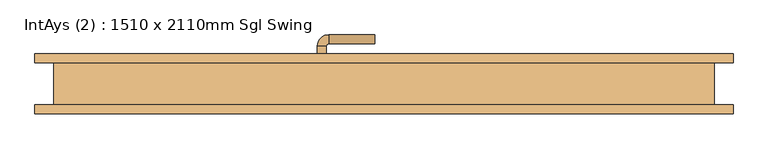
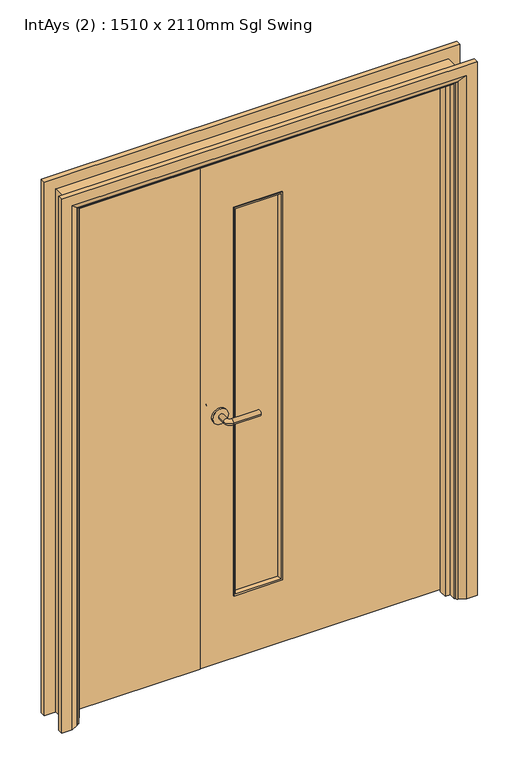
"""IFC4 building model written with IfcOpenShell, lengths in millimetres: door geometry, IntAys (2) : 1510 x 2110mm Sgl Swing."""

from ifc_helpers import new_model, si_unit, point, frame, frame_2d, origin, place, context, project, spatial, polyline, circle_curve, ellipse_curve, trimmed, segment, composite_curve, outline, extrude, faceted_brep, source, transform, mapped, element, save
from ifc_brep_helpers import plane_surface, cylinder_surface, revolved_surface, advanced_brep


def intays_2_1510_x_2110mm_sgl_swing_f165abe8(model_context):
    return source(origin(), model_context, "Body", "SolidModel", [
        advanced_brep(
        [(88.5, 7.5, 1000.0), (108.5, 7.5, 1000.0), (108.5, -22.5, 1000.0), (88.5, -22.5, 1000.0), (113.5, -27.5, 1000.0), (113.5, -47.5, 1000.0), (218.5, -47.5, 1000.0), (218.5, -27.5, 1000.0)],
        [
            (0, 1, circle_curve(frame((98.5, 7.5, 1000.0), z_axis=(0.0, 1.0, 0.0), x_axis=(1.0, 0.0, 0.0)), 10.0)),
            (1, 0, circle_curve(frame((98.5, 7.5, 1000.0), z_axis=(0.0, 1.0, 0.0), x_axis=(1.0, 0.0, 0.0)), 10.0)),
            (1, 2),
            (2, 3, circle_curve(frame((98.5, -22.5, 1000.0), z_axis=(0.0, 1.0, 0.0), x_axis=(1.0, 0.0, 0.0)), 10.0)),
            (3, 0),
            (3, 2, circle_curve(frame((98.5, -22.5, 1000.0), z_axis=(0.0, 1.0, 0.0), x_axis=(1.0, 0.0, 0.0)), 10.0)),
            (4, 5, circle_curve(frame((113.5, -37.5, 1000.0), z_axis=(-1.0, 0.0, 0.0), x_axis=(0.0, 1.0, 0.0)), 10.0)),
            (5, 3, circle_curve(frame((113.5, -22.5, 1000.0), z_axis=(0.0, 0.0, -1.0), x_axis=(-1.0, 0.0, 0.0)), 25.0)),
            (2, 4, circle_curve(frame((113.5, -22.5, 1000.0), z_axis=(0.0, 0.0, 1.0), x_axis=(-1.0, 0.0, 0.0)), 5.0)),
            (5, 4, circle_curve(frame((113.5, -37.5, 1000.0), z_axis=(-1.0, 0.0, 0.0), x_axis=(0.0, 1.0, 0.0)), 10.0)),
            (6, 7, circle_curve(frame((218.5, -37.5, 1000.0), z_axis=(1.0, 0.0, 0.0), x_axis=(0.0, 1.0, 0.0)), 10.0)),
            (7, 6, circle_curve(frame((218.5, -37.5, 1000.0), z_axis=(1.0, 0.0, 0.0), x_axis=(0.0, 1.0, 0.0)), 10.0)),
            (4, 7),
            (6, 5),
        ],
        [
            plane_surface(frame((98.5, 7.5, 1000.0), z_axis=(0.0, 1.0, 0.0), x_axis=(0.0, 0.0, 1.0))),
            cylinder_surface(frame((98.5, 7.5, 1000.0), z_axis=(0.0, 1.0, 0.0), x_axis=(1.0, 0.0, 0.0)), 10.0),
            revolved_surface(trimmed(ellipse_curve(frame((98.5, -22.5, 1000.0), z_axis=(0.0, -1.0, 0.0), x_axis=(1.0, 0.0, 0.0)), 10.0, 10.0), [point((88.5, -22.5, 1000.0))], [point((108.5, -22.5, 1000.0))], True, "CARTESIAN"), (113.5, -22.5, 1000.0), (0.0, 0.0, -1.0)),
            revolved_surface(trimmed(ellipse_curve(frame((98.5, -22.5, 1000.0), z_axis=(0.0, -1.0, 0.0), x_axis=(1.0, 0.0, 0.0)), 10.0, 10.0), [point((108.5, -22.5, 1000.0))], [point((88.5, -22.5, 1000.0))], True, "CARTESIAN"), (113.5, -22.5, 1000.0), (0.0, 0.0, -1.0)),
            plane_surface(frame((218.5, -37.5, 1000.0), z_axis=(1.0, 0.0, 0.0), x_axis=(0.0, 0.0, 1.0))),
            cylinder_surface(frame((113.5, -37.5, 1000.0), z_axis=(-1.0, 0.0, 0.0), x_axis=(0.0, 1.0, 0.0)), 10.0),
        ],
        [
            (0, [[1, 2]]),
            (1, [[3, 4, 5, -2]]),
            (1, [[-5, 6, -3, -1]]),
            (2, [[7, 8, -4, 9]]),
            (3, [[10, -9, -6, -8]]),
            (4, [[11, 12]]),
            (5, [[13, -11, 14, -7]]),
            (5, [[-14, -12, -13, -10]]),
        ],
    ),
        extrude(outline(composite_curve([segment(trimmed(circle_curve(frame_2d((1000.0, 96.0)), 30.0), [point((1000.0, 66.0))], [point((1000.0, 126.0))], False, "CARTESIAN"), True, "CONTINUOUS"), segment(trimmed(circle_curve(frame_2d((1000.0, 96.0)), 30.0), [point((1000.0, 126.0))], [point((1000.0, 66.0))], False, "CARTESIAN"), True, "CONTINUOUS")], self_intersect=False)), frame((0.0, 7.5, 0.0), z_axis=(0.0, 1.0, 0.0), x_axis=(0.0, 0.0, 1.0)), (0.0, 0.0, 1.0), 8.0),
        advanced_brep(
        [(88.5, 55.5, 1000.0), (108.5, 55.5, 1000.0), (88.5, 85.5, 1000.0), (108.5, 85.5, 1000.0), (113.5, 90.5, 1000.0), (113.5, 110.5, 1000.0), (218.5, 110.5, 1000.0), (218.5, 90.5, 1000.0)],
        [
            (0, 1, circle_curve(frame((98.5, 55.5, 1000.0), z_axis=(0.0, -1.0, 0.0), x_axis=(1.0, 0.0, 0.0)), 10.0)),
            (1, 0, circle_curve(frame((98.5, 55.5, 1000.0), z_axis=(0.0, -1.0, 0.0), x_axis=(1.0, 0.0, 0.0)), 10.0)),
            (0, 2),
            (2, 3, circle_curve(frame((98.5, 85.5, 1000.0), z_axis=(0.0, -1.0, 0.0), x_axis=(1.0, 0.0, 0.0)), 10.0)),
            (3, 1),
            (3, 2, circle_curve(frame((98.5, 85.5, 1000.0), z_axis=(0.0, -1.0, 0.0), x_axis=(1.0, 0.0, 0.0)), 10.0)),
            (4, 3, circle_curve(frame((113.5, 85.5, 1000.0), z_axis=(0.0, 0.0, 1.0), x_axis=(-1.0, 0.0, 0.0)), 5.0)),
            (2, 5, circle_curve(frame((113.5, 85.5, 1000.0), z_axis=(0.0, 0.0, -1.0), x_axis=(-1.0, 0.0, 0.0)), 25.0)),
            (5, 4, circle_curve(frame((113.5, 100.5, 1000.0), z_axis=(-1.0, 0.0, 0.0), x_axis=(0.0, -1.0, 0.0)), 10.0)),
            (4, 5, circle_curve(frame((113.5, 100.5, 1000.0), z_axis=(-1.0, 0.0, 0.0), x_axis=(0.0, -1.0, 0.0)), 10.0)),
            (6, 7, circle_curve(frame((218.5, 100.5, 1000.0), z_axis=(1.0, 0.0, 0.0), x_axis=(0.0, -1.0, 0.0)), 10.0)),
            (7, 6, circle_curve(frame((218.5, 100.5, 1000.0), z_axis=(1.0, 0.0, 0.0), x_axis=(0.0, -1.0, 0.0)), 10.0)),
            (5, 6),
            (7, 4),
        ],
        [
            plane_surface(frame((98.5, 55.5, 1000.0), z_axis=(0.0, -1.0, 0.0), x_axis=(0.0, 0.0, 1.0))),
            cylinder_surface(frame((98.5, 55.5, 1000.0), z_axis=(0.0, -1.0, 0.0), x_axis=(1.0, 0.0, 0.0)), 10.0),
            revolved_surface(trimmed(ellipse_curve(frame((98.5, 85.5, 1000.0), z_axis=(0.0, -1.0, 0.0), x_axis=(1.0, 0.0, 0.0)), 10.0, 10.0), [point((88.5, 85.5, 1000.0))], [point((108.5, 85.5, 1000.0))], True, "CARTESIAN"), (113.5, 85.5, 1000.0), (0.0, 0.0, -1.0)),
            revolved_surface(trimmed(ellipse_curve(frame((98.5, 85.5, 1000.0), z_axis=(0.0, -1.0, 0.0), x_axis=(1.0, 0.0, 0.0)), 10.0, 10.0), [point((108.5, 85.5, 1000.0))], [point((88.5, 85.5, 1000.0))], True, "CARTESIAN"), (113.5, 85.5, 1000.0), (0.0, 0.0, -1.0)),
            plane_surface(frame((218.5, 100.5, 1000.0), z_axis=(1.0, 0.0, 0.0), x_axis=(0.0, 0.0, 1.0))),
            cylinder_surface(frame((113.5, 100.5, 1000.0), z_axis=(-1.0, 0.0, 0.0), x_axis=(0.0, -1.0, 0.0)), 10.0),
        ],
        [
            (0, [[1, 2]]),
            (1, [[-1, 3, 4, 5]]),
            (1, [[-2, -5, 6, -3]]),
            (2, [[7, -4, 8, 9]]),
            (3, [[-8, -6, -7, 10]]),
            (4, [[11, 12]]),
            (5, [[-9, 13, -12, 14]]),
            (5, [[-10, -14, -11, -13]]),
        ],
    ),
        extrude(outline(composite_curve([segment(trimmed(circle_curve(frame_2d((1000.0, 96.0)), 30.0), [point((1000.0, 66.0))], [point((1000.0, 126.0))], False, "CARTESIAN"), True, "CONTINUOUS"), segment(trimmed(circle_curve(frame_2d((1000.0, 96.0)), 30.0), [point((1000.0, 126.0))], [point((1000.0, 66.0))], False, "CARTESIAN"), True, "CONTINUOUS")], self_intersect=False)), frame((0.0, 47.5, 0.0), z_axis=(0.0, 1.0, 0.0), x_axis=(0.0, 0.0, 1.0)), (0.0, 0.0, 1.0), 8.0),
        extrude(outline(polyline([(2102.0, -508.0), (0.0, -508.0), (0.0, -476.0), (2070.0, -476.0), (2070.0, 954.0), (0.0, 954.0), (0.0, 986.0), (2102.0, 986.0), (2102.0, -508.0)])), frame((0.0, -47.5, 0.0), z_axis=(0.0, 1.0, 0.0), x_axis=(0.0, 0.0, 1.0)), (0.0, 0.0, 1.0), 95.0),
        advanced_brep(
        [(-551.0, -67.5, 0.0), (-551.0, -47.5, 0.0), (-481.0, -47.5, 0.0), (-485.0, -53.5, 0.0), (-511.0, -67.5, 0.0), (-551.0, -67.5, 2145.0), (-551.0, -47.5, 2145.0), (1029.0, -47.5, 2145.0), (1029.0, -47.5, 0.0), (959.0, -47.5, 0.0), (959.0, -47.5, 2075.0), (-481.0, -47.5, 2075.0), (-485.0, -53.5, 2079.0), (-511.0, -67.5, 2105.0), (989.0, -67.5, 2105.0), (989.0, -67.5, 0.0), (1029.0, -67.5, 0.0), (1029.0, -67.5, 2145.0), (963.0, -53.5, 0.0), (963.0, -53.5, 2079.0)],
        [
            (0, 1),
            (1, 2),
            (2, 3, circle_curve(frame((-489.0, -46.5, 0.0), z_axis=(0.0, 0.0, -1.0), x_axis=(-1.0, 0.0, 0.0)), 8.0622577)),
            (3, 4),
            (4, 0),
            (0, 5),
            (5, 6),
            (6, 1),
            (6, 7),
            (7, 8),
            (8, 9),
            (9, 10),
            (10, 11),
            (11, 2),
            (11, 12, ellipse_curve(frame((-489.0, -46.5, 2083.0), z_axis=(-0.7071067811865475, 0.0, -0.7071067811865475), x_axis=(0.7071067811865474, 0.0, -0.7071067811865476)), 11.4017543, 8.0622577)),
            (12, 3),
            (12, 13),
            (13, 4),
            (13, 14),
            (14, 15),
            (15, 16),
            (16, 17),
            (17, 5),
            (7, 17),
            (16, 8),
            (15, 18),
            (18, 9, circle_curve(frame((967.0, -46.5, 0.0), z_axis=(0.0, 0.0, -1.0), x_axis=(1.0, 0.0, 0.0)), 8.0622577)),
            (19, 10, ellipse_curve(frame((967.0, -46.5, 2083.0), z_axis=(0.7071067811865475, 0.0, -0.7071067811865475), x_axis=(0.7071067811865474, 0.0, 0.7071067811865476)), 11.4017543, 8.0622577)),
            (18, 19),
            (14, 19),
            (19, 12),
        ],
        [
            plane_surface(frame((-481.0, -47.5, 0.0), z_axis=(0.0, 0.0, -1.0), x_axis=(0.0, -1.0, 0.0))),
            plane_surface(frame((-551.0, -67.5, 0.0), z_axis=(-1.0, 0.0, 0.0), x_axis=(0.0, 0.0, 1.0))),
            plane_surface(frame((-551.0, -47.5, 0.0), z_axis=(0.0, 1.0, 0.0), x_axis=(0.0, 0.0, 1.0))),
            cylinder_surface(frame((-489.0, -46.5, 0.0), z_axis=(0.0, 0.0, -1.0), x_axis=(-1.0, 0.0, 0.0)), 8.0622577),
            plane_surface(frame((-485.0, -53.5, 0.0), z_axis=(0.4740998230350183, -0.8804710999221749, 0.0), x_axis=(0.0, 0.0, 1.0))),
            plane_surface(frame((-511.0, -67.5, 0.0), z_axis=(0.0, -1.0, 0.0), x_axis=(0.0, 0.0, 1.0))),
            plane_surface(frame((1029.0, -67.5, 2145.0), z_axis=(1.0, 0.0, 0.0), x_axis=(0.0, 0.0, -1.0))),
            plane_surface(frame((959.0, -47.5, 0.0), z_axis=(0.0, 0.0, -1.0), x_axis=(0.0, -1.0, 0.0))),
            cylinder_surface(frame((967.0, -46.5, 2075.0), z_axis=(0.0, 0.0, 1.0), x_axis=(1.0, 0.0, 0.0)), 8.0622577),
            plane_surface(frame((963.0, -53.5, 2079.0), z_axis=(-0.4740998230350183, -0.8804710999221749, 0.0), x_axis=(0.0, 0.0, -1.0))),
            plane_surface(frame((-551.0, -67.5, 2145.0), z_axis=(0.0, 0.0, 1.0), x_axis=(1.0, 0.0, 0.0))),
            cylinder_surface(frame((-481.0, -46.5, 2083.0), z_axis=(-1.0, 0.0, 0.0), x_axis=(0.0, 0.0, 1.0)), 8.0622577),
            plane_surface(frame((-485.0, -53.5, 2079.0), z_axis=(0.0, -0.8804710999221749, -0.4740998230350183), x_axis=(1.0, 0.0, 0.0))),
        ],
        [
            (0, [[1, 2, 3, 4, 5]]),
            (1, [[-1, 6, 7, 8]]),
            (2, [[-2, -8, 9, 10, 11, 12, 13, 14]]),
            (3, [[-3, -14, 15, 16]]),
            (4, [[-4, -16, 17, 18]]),
            (5, [[-5, -18, 19, 20, 21, 22, 23, -6]]),
            (6, [[24, -22, 25, -10]]),
            (7, [[-21, 26, 27, -11, -25]]),
            (8, [[28, -12, -27, 29]]),
            (9, [[30, -29, -26, -20]]),
            (10, [[-7, -23, -24, -9]]),
            (11, [[-15, -13, -28, 31]]),
            (12, [[-17, -31, -30, -19]]),
        ],
    ),
        advanced_brep(
        [(1029.0, 67.5, 0.0), (1029.0, 47.5, 0.0), (959.0, 47.5, 0.0), (963.0, 53.5, 0.0), (989.0, 67.5, 0.0), (1029.0, 67.5, 2145.0), (1029.0, 47.5, 2145.0), (-551.0, 47.5, 2145.0), (-551.0, 47.5, 0.0), (-481.0, 47.5, 0.0), (-481.0, 47.5, 2075.0), (959.0, 47.5, 2075.0), (963.0, 53.5, 2079.0), (989.0, 67.5, 2105.0), (-511.0, 67.5, 2105.0), (-511.0, 67.5, 0.0), (-551.0, 67.5, 0.0), (-551.0, 67.5, 2145.0), (-485.0, 53.5, 0.0), (-485.0, 53.5, 2079.0)],
        [
            (0, 1),
            (1, 2),
            (2, 3, circle_curve(frame((967.0, 46.5, 0.0), z_axis=(0.0, 0.0, -1.0), x_axis=(1.0, 0.0, 0.0)), 8.0622577)),
            (3, 4),
            (4, 0),
            (0, 5),
            (5, 6),
            (6, 1),
            (6, 7),
            (7, 8),
            (8, 9),
            (9, 10),
            (10, 11),
            (11, 2),
            (11, 12, ellipse_curve(frame((967.0, 46.5, 2083.0), z_axis=(0.7071067811865475, 0.0, -0.7071067811865475), x_axis=(-0.7071067811865474, 0.0, -0.7071067811865476)), 11.4017543, 8.0622577)),
            (12, 3),
            (12, 13),
            (13, 4),
            (13, 14),
            (14, 15),
            (15, 16),
            (16, 17),
            (17, 5),
            (7, 17),
            (16, 8),
            (15, 18),
            (18, 9, circle_curve(frame((-489.0, 46.5, 0.0), z_axis=(0.0, 0.0, -1.0), x_axis=(-1.0, 0.0, 0.0)), 8.0622577)),
            (19, 10, ellipse_curve(frame((-489.0, 46.5, 2083.0), z_axis=(-0.7071067811865475, 0.0, -0.7071067811865475), x_axis=(-0.7071067811865474, 0.0, 0.7071067811865476)), 11.4017543, 8.0622577)),
            (18, 19),
            (14, 19),
            (19, 12),
        ],
        [
            plane_surface(frame((959.0, 47.5, 0.0), z_axis=(0.0, 0.0, -1.0), x_axis=(0.0, -1.0, 0.0))),
            plane_surface(frame((1029.0, 67.5, 0.0), z_axis=(1.0, 0.0, 0.0), x_axis=(0.0, 0.0, 1.0))),
            plane_surface(frame((1029.0, 47.5, 0.0), z_axis=(0.0, -1.0, 0.0), x_axis=(0.0, 0.0, 1.0))),
            cylinder_surface(frame((967.0, 46.5, 0.0), z_axis=(0.0, 0.0, -1.0), x_axis=(1.0, 0.0, 0.0)), 8.0622577),
            plane_surface(frame((963.0, 53.5, 0.0), z_axis=(-0.4740998230350126, 0.8804710999221779, 0.0), x_axis=(0.0, 0.0, 1.0))),
            plane_surface(frame((989.0, 67.5, 0.0), z_axis=(0.0, 1.0, 0.0), x_axis=(0.0, 0.0, 1.0))),
            plane_surface(frame((-551.0, 67.5, 2145.0), z_axis=(-1.0, 0.0, 0.0), x_axis=(0.0, 0.0, -1.0))),
            plane_surface(frame((-481.0, 47.5, 0.0), z_axis=(0.0, 0.0, -1.0), x_axis=(0.0, -1.0, 0.0))),
            cylinder_surface(frame((-489.0, 46.5, 2075.0), z_axis=(0.0, 0.0, 1.0), x_axis=(-1.0, 0.0, 0.0)), 8.0622577),
            plane_surface(frame((-485.0, 53.5, 2079.0), z_axis=(0.4740998230350183, 0.8804710999221749, 0.0), x_axis=(0.0, 0.0, -1.0))),
            plane_surface(frame((1029.0, 67.5, 2145.0), z_axis=(0.0, 0.0, 1.0), x_axis=(-1.0, 0.0, 0.0))),
            cylinder_surface(frame((959.0, 46.5, 2083.0), z_axis=(1.0, 0.0, 0.0), x_axis=(0.0, 0.0, 1.0)), 8.0622577),
            plane_surface(frame((963.0, 53.5, 2079.0), z_axis=(0.0, 0.8804710999221763, -0.4740998230350154), x_axis=(-1.0, 0.0, 0.0))),
        ],
        [
            (0, [[1, 2, 3, 4, 5]]),
            (1, [[-1, 6, 7, 8]]),
            (2, [[-2, -8, 9, 10, 11, 12, 13, 14]]),
            (3, [[-3, -14, 15, 16]]),
            (4, [[-4, -16, 17, 18]]),
            (5, [[-5, -18, 19, 20, 21, 22, 23, -6]]),
            (6, [[24, -22, 25, -10]]),
            (7, [[-21, 26, 27, -11, -25]]),
            (8, [[28, -12, -27, 29]]),
            (9, [[30, -29, -26, -20]]),
            (10, [[-7, -23, -24, -9]]),
            (11, [[-15, -13, -28, 31]]),
            (12, [[-17, -31, -30, -19]]),
        ],
    ),
        faceted_brep([(-457.0, 12.5, 0.0), (-457.0, -19.5, 0.0), (-476.0, -19.5, 0.0), (-476.0, 12.5, 0.0), (-457.0, 12.5, 2051.0), (-457.0, -19.5, 2051.0), (-476.0, -19.5, 2070.0), (-476.0, 12.5, 2070.0), (935.0, 12.5, 0.0), (954.0, 12.5, 0.0), (954.0, -19.5, 0.0), (935.0, -19.5, 0.0), (935.0, 12.5, 2051.0), (954.0, 12.5, 2070.0), (954.0, -19.5, 2070.0), (935.0, -19.5, 2051.0)], [[[0, 1, 2, 3]], [[1, 0, 4, 5]], [[2, 1, 5, 6]], [[3, 2, 6, 7]], [[0, 3, 7, 4]], [[8, 9, 10, 11]], [[12, 13, 9, 8]], [[13, 14, 10, 9]], [[14, 15, 11, 10]], [[15, 12, 8, 11]], [[5, 4, 12, 15]], [[6, 5, 15, 14]], [[7, 6, 14, 13]], [[4, 7, 13, 12]]]),
        extrude(outline(polyline([(335.0, 25.5), (150.0, 25.5), (150.0, 37.5), (335.0, 37.5), (335.0, 25.5)])), frame((0.0, 0.0, 257.0), z_axis=(0.0, 0.0, 1.0), x_axis=(1.0, 0.0, 0.0)), (0.0, 0.0, 1.0), 1560.0),
        extrude(outline(polyline([(22.0, 15.5), (-473.0, 15.5), (-473.0, 47.5), (22.0, 47.5), (22.0, 15.5)])), frame((0.0, 0.0, 5.753223), z_axis=(0.0, 0.0, 1.0), x_axis=(1.0, 0.0, 0.0)), (0.0, 0.0, 1.0), 2061.246777),
        extrude(outline(polyline([(5.753223, 951.0), (2067.0, 951.0), (2067.0, 25.0), (5.753223, 25.0), (5.753223, 951.0)]), holes=[polyline([(1817.0, 150.0), (1817.0, 335.0), (257.0, 335.0), (257.0, 150.0), (1817.0, 150.0)])]), frame((0.0, 15.5, 0.0), z_axis=(0.0, 1.0, 0.0), x_axis=(0.0, 0.0, 1.0)), (0.0, 0.0, 1.0), 32.0),
        faceted_brep([(335.0, 12.5, 257.0), (335.0, 25.5, 257.0), (335.0, 25.5, 1817.0), (335.0, 12.5, 1817.0), (323.0, 25.5, 269.0), (329.0, 12.5, 263.0), (329.0, 12.5, 1811.0), (323.0, 25.5, 1805.0), (150.0, 25.5, 1817.0), (150.0, 12.5, 1817.0), (156.0, 12.5, 1811.0), (162.0, 25.5, 1805.0), (150.0, 25.5, 257.0), (150.0, 12.5, 257.0), (156.0, 12.5, 263.0), (162.0, 25.5, 269.0)], [[[0, 1, 2, 3]], [[4, 5, 6, 7]], [[3, 2, 8, 9]], [[7, 6, 10, 11]], [[9, 8, 12, 13]], [[11, 10, 14, 15]], [[1, 12, 8, 2], [7, 11, 15, 4]], [[13, 12, 1, 0]], [[3, 9, 13, 0], [5, 14, 10, 6]], [[15, 14, 5, 4]]]),
        faceted_brep([(150.0, 50.5, 257.0), (150.0, 37.5, 257.0), (150.0, 37.5, 1817.0), (150.0, 50.5, 1817.0), (162.0, 37.5, 269.0), (156.0, 50.5, 263.0), (156.0, 50.5, 1811.0), (162.0, 37.5, 1805.0), (335.0, 37.5, 1817.0), (335.0, 50.5, 1817.0), (329.0, 50.5, 1811.0), (323.0, 37.5, 1805.0), (335.0, 37.5, 257.0), (335.0, 50.5, 257.0), (329.0, 50.5, 263.0), (323.0, 37.5, 269.0)], [[[0, 1, 2, 3]], [[4, 5, 6, 7]], [[3, 2, 8, 9]], [[7, 6, 10, 11]], [[9, 8, 12, 13]], [[11, 10, 14, 15]], [[1, 12, 8, 2], [7, 11, 15, 4]], [[13, 12, 1, 0]], [[3, 9, 13, 0], [5, 14, 10, 6]], [[15, 14, 5, 4]]]),
    ])


if __name__ == "__main__":
    model = new_model("IFC4")
    model_context = context("Model", 3, world=origin())
    ifc_project = project(units=[si_unit("LENGTHUNIT", "METRE", prefix="MILLI")], contexts=[model_context])
    site = spatial("IfcSite", under=ifc_project)
    building = spatial("IfcBuilding", under=site)
    placement = place(None, origin())
    intays_2_1510_x_2110mm_sgl_swing_shape = intays_2_1510_x_2110mm_sgl_swing_f165abe8(model_context)
    element("IfcDoor", 1, ObjectType="IntAys (2) : 1510 x 2110mm Sgl Swing", at=placement, inside=building, context=model_context, shape_type="MappedRepresentation", body=[
        mapped(intays_2_1510_x_2110mm_sgl_swing_shape, transform((0.0, 0.0, 0.0), x_axis=(1.0, 0.0, 0.0), y_axis=(0.0, 1.0, 0.0), z_axis=(0.0, 0.0, 1.0))),
    ])
    save(model, "model.ifc")

# Revit data of these elements
# Type "IntAys (2) : 1510 x 2110mm Sgl Swing"
#   Type Mark = "46"
#   Type Comments = "Internal Asymmetric"
#   Operation = "DoubleDoorSingleSwing"
#   Construction Type Id = "SGL"
#   Keynote = "L20"
#   Description = "Internal Asymmetric Door"
#   Analytic Construction = "Large single-glazed windows"
#   Visual Light Transmittance = 0.9
#   VisionPanel Width = 185 mm
#   Thickness = 32 mm
#   Stop Thickness = 19 mm
#   Stop Depth = 32 mm
#   Stile Top Rail = 250 mm
#   Stile Shutting = 125 mm
#   Stile Bottom Rail = 250 mm
#   Solar Heat Gain Coefficient = 0.86
#   Secondary Panel Width = 495 mm
#   Rough Width = 1510 mm
#   Rough Height = 2110 mm
#   Main Panel Width = 926 mm
#   Heat Transfer Coefficient (U) = 5.5617 W/(m²·K)
#   Handle Z Distance = 1000 mm
#   Handle X Distance = 75 mm
#   Handle Length = 350 mm
#   Frame Thickness = 32 mm
#   Door Panel Width = 926 mm
#   Door Panel Thickness = 32 mm
#   Height = 2110 mm
#   Door Panel Offset = 0 mm
#   Structural Tolerance = 8 mm
#   Tolerance = 3 mm
#   UnderCut = 7 mm
#   Width = 1510 mm
#   Door Panel Height = 2060 mm
#   Architrave Setback = 5 mm
#   Vis - Swing Single = yes
#   Vis - Swing Opposing = no
#   Vis - Swing Double = no
#   Vis - Stops = yes
#   Vis - Ironmongery = yes
#   Define Thermal Properties by = 1
#   Material Ironmongery = Door - Handle
#   Material Glass = Door - Glazing
#   Material Frame = Door - Frame/Mullion
#   Material Door = Door - Panel
#   Material Beading = Door - Panel
#   Material Architrave = Door - Architrave
#   Handle Style = element 261135
#   Function = (empty or 0)
#   Wall Closure = (empty or 0)
# Element 1 (IfcDoor, "IntAys (2) : 1510 x 2110mm Sgl Swing")
#   Materials on its faces: "Door - Panel", "Door - Architrave", "Door - Handle", "Door - Frame/Mullion", "Door - Glazing"
# Materials
#   "Door - Handle": class "Miscellaneous", colour RGB 0 0 0, transparency 0, Keynote = "P21"
#   "Door - Glazing": class "Miscellaneous", colour RGB 0 0 255, transparency 0.75
#   "Door - Frame/Mullion": class "Wood", colour RGB 212 179 113, transparency 0, Keynote = "L20"
#   "Door - Panel": class "Wood", colour RGB 210 159 95, transparency 0, Keynote = "L20"
#   "Door - Architrave": class "Wood", colour RGB 154 90 5, transparency 0, Keynote = "P20"
